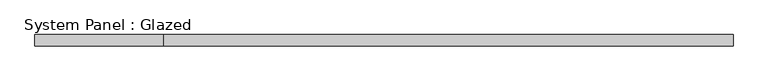
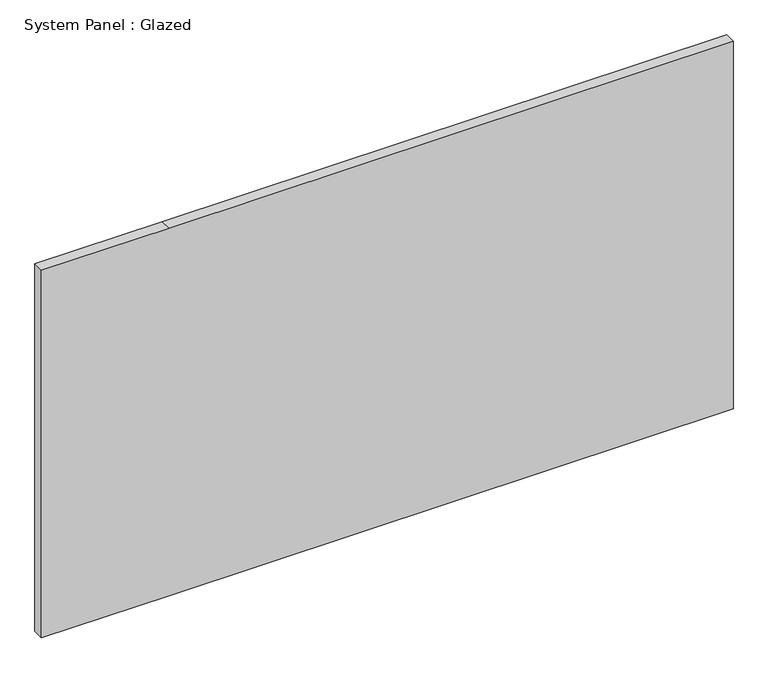
"""IFC4 building model written with IfcOpenShell, lengths in millimetres: plate geometry, System Panel : Glazed."""

from ifc_helpers import new_model, si_unit, frame, origin, place, context, project, spatial, polyline, outline, extrude, source, transform, mapped, element, save


def system_panel_glazed_3fe504bb(model_context):
    return source(origin(), model_context, "Body", "SweptSolid", [
        extrude(outline(polyline([(0.0, -774.7), (0.0, -488.95), (0.0, 774.7), (869.95, 774.7), (869.95, -488.95), (869.95, -774.7), (0.0, -774.7)])), frame((0.0, 19.05, 0.0), z_axis=(0.0, 1.0, 0.0), x_axis=(0.0, 0.0, 1.0)), (0.0, 0.0, 1.0), 25.4),
    ])


if __name__ == "__main__":
    model = new_model("IFC4")
    model_context = context("Model", 3, world=origin())
    ifc_project = project(units=[si_unit("LENGTHUNIT", "METRE", prefix="MILLI")], contexts=[model_context])
    site = spatial("IfcSite", under=ifc_project)
    building = spatial("IfcBuilding", under=site)
    placement = place(None, origin())
    system_panel_glazed_shape = system_panel_glazed_3fe504bb(model_context)
    element("IfcPlate", 1, ObjectType="System Panel : Glazed", at=placement, inside=building, context=model_context, shape_type="MappedRepresentation", body=[
        mapped(system_panel_glazed_shape, transform((0.0, 0.0, 0.0), x_axis=(1.0, 0.0, 0.0), y_axis=(0.0, 1.0, 0.0), z_axis=(0.0, 0.0, 1.0))),
    ])
    save(model, "model.ifc")

# Revit data of these elements
# Element 1 (IfcPlate, "System Panel : Glazed")
#   Materials on its faces: "Glass"
# Materials
#   "Glass": class "Glass", colour RGB 0 128 192, transparency 0.75
